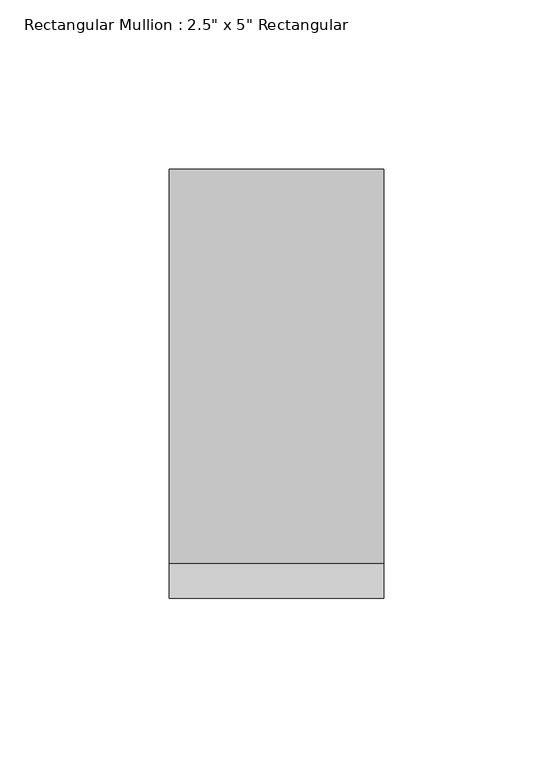
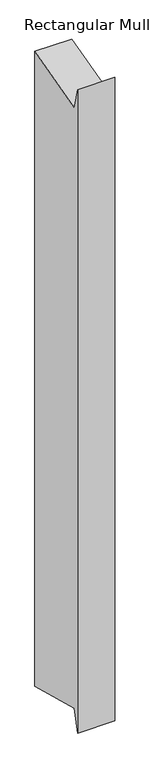
"""IFC4 building model written with IfcOpenShell, lengths in millimetres: member geometry."""

import ifcopenshell
import ifcopenshell.guid

model = None  # the IFC model being written
_history = None  # IfcOwnerHistory: only IFC2X3 demands one
_inside = {}  # id of a spatial element -> (the spatial element, [elements in it])
_under = {}  # id of a project, library or spatial element -> (it, [spatial elements below it])
_declared = {}  # id of a project -> (the project, [libraries it declares])
_typed = {}  # id of a type object -> (the type object, [elements of that type])
_made_of = {}  # id of a material, layer set ... -> (it, [elements and type objects made of it])


def new_model(schema):
    """Start an empty IFC model of exactly this schema.

    Asked for "IFC4X3", IfcOpenShell would pick the latest addendum, in which some entities
    have other attributes; the version numbers below select the first issue.
    IFC2X3 requires an IfcOwnerHistory on every rooted entity: one is made here for all.
    """
    global model, _history
    if schema == "IFC4X3":
        model = ifcopenshell.file(schema_version=(4, 3, 0, 0))
    else:
        model = ifcopenshell.file(schema=schema)
    _inside.clear()
    _under.clear()
    _declared.clear()
    _typed.clear()
    _made_of.clear()
    _history = None
    if model.schema == "IFC2X3":
        org = make("IfcOrganization", Name="unknown")
        user = make(
            "IfcPersonAndOrganization",
            ThePerson=make("IfcPerson", FamilyName="unknown"),
            TheOrganization=org,
        )
        app = make(
            "IfcApplication",
            ApplicationDeveloper=org,
            Version="unknown",
            ApplicationFullName="unknown",
            ApplicationIdentifier="unknown",
        )
        _history = make(
            "IfcOwnerHistory",
            OwningUser=user,
            OwningApplication=app,
            ChangeAction="ADDED",
            CreationDate=0,
        )
    return model


def make(cls, **values):
    """One entity of the class cls with the attributes given. An attribute that is None is left unset."""
    return model.create_entity(
        cls, **{name: value for name, value in values.items() if value is not None}
    )


def rooted(cls, **values):
    """An entity with a GlobalId (a new one), such as an element, a storey or a relation."""
    return make(cls, GlobalId=ifcopenshell.guid.new(), OwnerHistory=_history, **values)


def si_unit(unit_type, name, prefix=None):
    """IfcSIUnit, for example si_unit("LENGTHUNIT", "METRE", prefix="MILLI")."""
    return make("IfcSIUnit", UnitType=unit_type, Prefix=prefix, Name=name)


def assignment(units):
    """IfcUnitAssignment: the units of a project."""
    return None if units is None else make("IfcUnitAssignment", Units=units)


def point(xyz):
    """IfcCartesianPoint."""
    return None if xyz is None else make("IfcCartesianPoint", Coordinates=xyz)


def direction(xyz):
    """IfcDirection."""
    return None if xyz is None else make("IfcDirection", DirectionRatios=xyz)


def frame(location, z_axis=None, x_axis=None):
    """IfcAxis2Placement3D, a coordinate frame: its origin and axes. An axis left out is left unset."""
    return make(
        "IfcAxis2Placement3D",
        Location=point(location),
        Axis=direction(z_axis),
        RefDirection=direction(x_axis),
    )


def origin():
    """The frame at (0, 0, 0) with its axes left unset."""
    return frame((0.0, 0.0, 0.0))


def place(relative_to, where):
    """IfcLocalPlacement: puts the frame where relative to a parent placement (None: the world)."""
    return make(
        "IfcLocalPlacement", PlacementRelTo=relative_to, RelativePlacement=where
    )


def context(
    kind, dimensions, precision=None, world=None, true_north=None, identifier=None
):
    """IfcGeometricRepresentationContext, for example the 3D "Model" context."""
    return make(
        "IfcGeometricRepresentationContext",
        ContextIdentifier=identifier,
        ContextType=kind,
        CoordinateSpaceDimension=dimensions,
        Precision=precision,
        WorldCoordinateSystem=world,
        TrueNorth=true_north,
    )


def project(units=None, contexts=None):
    """IfcProject with its units and contexts."""
    return rooted(
        "IfcProject",
        Name="project",
        RepresentationContexts=contexts,
        UnitsInContext=assignment(units),
    )


def spatial(cls, under=None, at=None, **own):
    """A site, building, storey or space (cls), placed at a placement, below another one or the project."""
    s = rooted(cls, ObjectPlacement=at, **own)
    if under is not None:
        _under.setdefault(under.id(), (under, []))[1].append(s)
    return s


def polyline(points):
    """IfcPolyline through the points."""
    return make("IfcPolyline", Points=[point(p) for p in points])


def outline(outer, holes=None, kind="AREA"):
    """IfcArbitraryClosedProfileDef: a profile drawn as a closed curve; with holes, ...WithVoids."""
    if holes is None:
        return make("IfcArbitraryClosedProfileDef", ProfileType=kind, OuterCurve=outer)
    return make(
        "IfcArbitraryProfileDefWithVoids",
        ProfileType=kind,
        OuterCurve=outer,
        InnerCurves=holes,
    )


def extrude(swept, where, along, depth):
    """IfcExtrudedAreaSolid: the profile swept, set in the frame where, extruded along a direction by depth."""
    return make(
        "IfcExtrudedAreaSolid",
        SweptArea=swept,
        Position=where,
        ExtrudedDirection=direction(along),
        Depth=depth,
    )


def shape(context_of_items, identifier, shape_type, items):
    """IfcShapeRepresentation: the items that make up one representation, for example the "Body"."""
    return make(
        "IfcShapeRepresentation",
        ContextOfItems=context_of_items,
        RepresentationIdentifier=identifier,
        RepresentationType=shape_type,
        Items=items,
    )


def source(mapping_origin, context_of_items, identifier, shape_type, items):
    """IfcRepresentationMap: a shape defined once, which mapped items show again and again."""
    return make(
        "IfcRepresentationMap",
        MappingOrigin=mapping_origin,
        MappedRepresentation=shape(context_of_items, identifier, shape_type, items),
    )


def transform(
    local_origin,
    x_axis=None,
    y_axis=None,
    z_axis=None,
    scale=None,
    scale2=None,
    scale3=None,
    uniform=True,
):
    """IfcCartesianTransformationOperator3D, or its non-uniform kind. x_axis, y_axis, z_axis: its Axis1, 2, 3."""
    if uniform:
        return make(
            "IfcCartesianTransformationOperator3D",
            Axis1=direction(x_axis),
            Axis2=direction(y_axis),
            LocalOrigin=point(local_origin),
            Scale=scale,
            Axis3=direction(z_axis),
        )
    return make(
        "IfcCartesianTransformationOperator3DnonUniform",
        Axis1=direction(x_axis),
        Axis2=direction(y_axis),
        LocalOrigin=point(local_origin),
        Scale=scale,
        Axis3=direction(z_axis),
        Scale2=scale2,
        Scale3=scale3,
    )


def mapped(mapping_source, mapping_target):
    """IfcMappedItem: shows the shape of a source again, moved by a transform."""
    return make(
        "IfcMappedItem", MappingSource=mapping_source, MappingTarget=mapping_target
    )


def made_of(thing, what):
    """Note that an element or type object is made of a material, layer set ...; save() writes the relation."""
    if what is not None:
        _made_of.setdefault(what.id(), (what, []))[1].append(thing)
    return thing


def element(
    cls,
    number,
    at=None,
    inside=None,
    cuts=None,
    type_object=None,
    material=None,
    context=None,
    identifier="Body",
    shape_type=None,
    held_by="IfcProductDefinitionShape",
    body=None,
    shapes=None,
    **own,
):
    """One element of the class cls, such as IfcWall. Its Tag is "e" and its number.

    at: its placement. inside: the storey or other place that contains it. cuts: it is an
    opening in that element (IfcRelVoidsElement). A single representation is given by context,
    identifier, shape_type and body (its items); several are given by shapes. held_by: the class
    of the entity that holds the representations. save() writes the other relations.
    """
    e = rooted(cls, Tag="e%d" % number, ObjectPlacement=at, **own)
    if body is not None:
        shapes = [shape(context, identifier, shape_type, body)]
    if shapes is not None:
        e.Representation = make(held_by, Representations=shapes)
    if inside is not None:
        _inside.setdefault(inside.id(), (inside, []))[1].append(e)
    if cuts is not None:
        rooted(
            "IfcRelVoidsElement", RelatingBuildingElement=cuts, RelatedOpeningElement=e
        )
    if type_object is not None:
        _typed.setdefault(type_object.id(), (type_object, []))[1].append(e)
    return made_of(e, material)


def aggregate(whole, parts):
    """IfcRelAggregates: a whole, such as a stair, and the parts it consists of."""
    return rooted("IfcRelAggregates", RelatingObject=whole, RelatedObjects=parts)


def save(model, path):
    """Write the relations noted so far, then the file.

    IfcRelAggregates (storeys below a building ...), IfcRelContainedInSpatialStructure (elements
    in a storey), IfcRelDefinesByType, IfcRelAssociatesMaterial and IfcRelDeclares: one each for
    every whole, place, type object, material and project.
    """
    for whole, parts in _under.values():
        aggregate(whole, parts)
    for where, things in _inside.values():
        rooted(
            "IfcRelContainedInSpatialStructure",
            RelatedElements=things,
            RelatingStructure=where,
        )
    for kind, things in _typed.values():
        rooted("IfcRelDefinesByType", RelatedObjects=things, RelatingType=kind)
    for what, things in _made_of.values():
        rooted("IfcRelAssociatesMaterial", RelatedObjects=things, RelatingMaterial=what)
    for by, libraries in _declared.values():
        rooted("IfcRelDeclares", RelatingContext=by, RelatedDefinitions=libraries)
    model.write(path)


def member_a3ab64da(model_context):
    return source(origin(), model_context, "Body", "SweptSolid", [
        extrude(outline(polyline([(-63.5, 23.3900664), (-53.1187853, -15.3531543), (63.5, 15.894755), (63.5, -1135.7154292), (-53.1187853, -1104.4675199), (-63.5, -1143.2107406), (-63.5, 23.3900664)])), frame((-63.5, 0.0, 0.0), z_axis=(1.0, 0.0, 0.0), x_axis=(0.0, 1.0, 0.0)), (0.0, 0.0, 1.0), 63.5),
    ])


if __name__ == "__main__":
    model = new_model("IFC4")
    model_context = context("Model", 3, world=origin())
    ifc_project = project(units=[si_unit("LENGTHUNIT", "METRE", prefix="MILLI")], contexts=[model_context])
    site = spatial("IfcSite", under=ifc_project)
    building = spatial("IfcBuilding", under=site)
    placement = place(None, origin())
    member_shape = member_a3ab64da(model_context)
    element("IfcMember", 1, ObjectType="Rectangular Mullion : 2.5\" x 5\" Rectangular", at=placement, inside=building, context=model_context, shape_type="MappedRepresentation", body=[
        mapped(member_shape, transform((0.0, 0.0, 0.0), x_axis=(1.0, 0.0, 0.0), y_axis=(0.0, 1.0, 0.0), z_axis=(0.0, 0.0, 1.0))),
    ])
    save(model, "model.ifc")

# Revit data of these elements
# Type "Rectangular Mullion : 2.5\" x 5\" Rectangular"
#   built-in parameter 1007304 = 0.416667 (stored number, unit not read)
#   built-in parameter 1007301 = 0.104167 (stored number, unit not read)
#   built-in parameter 1007300 = 0.104167 (stored number, unit not read)
# Element 1 (IfcMember, "Rectangular Mullion : 2.5\" x 5\" Rectangular")
#   Materials on its faces: "Aluminum"
# Materials
#   "Aluminum": class "Metal", colour RGB 247 247 247, transparency 0, Description = "Aluminum 6061", Cost = 0
